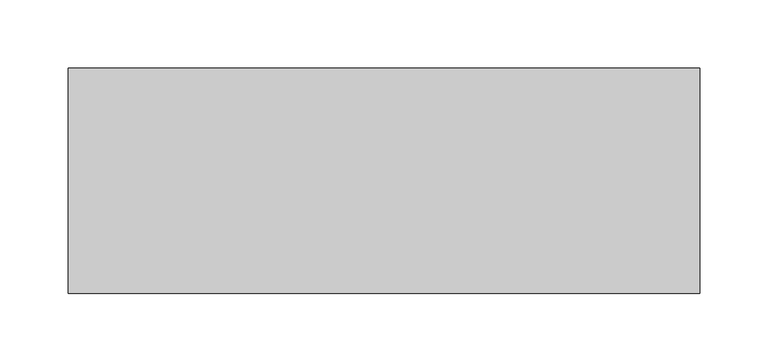
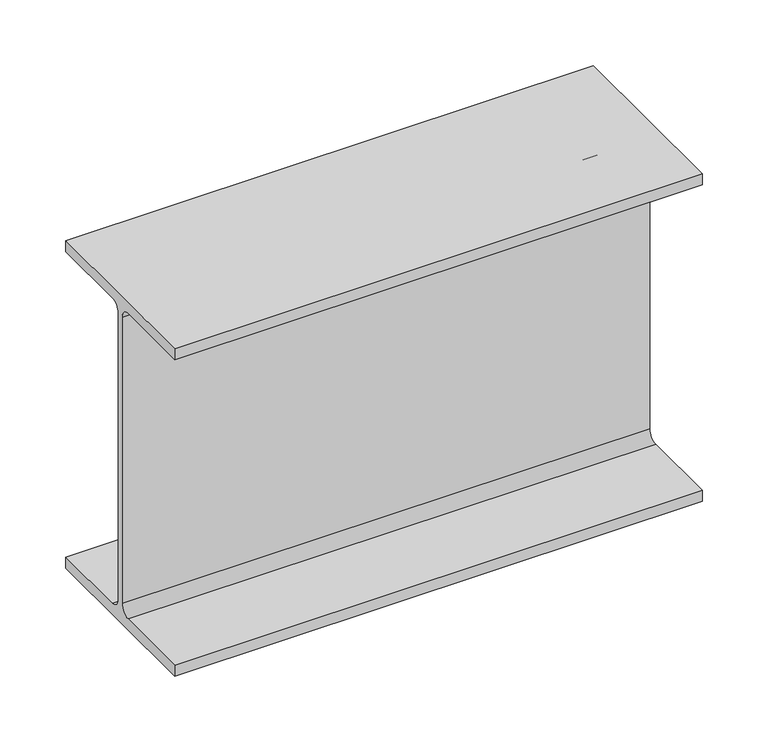
"""IFC4 building model written with IfcOpenShell, lengths in millimetres: beam geometry, Steel Beam_H-KSD3502 : H_SB_ASB_H-300x150x6.5x9."""

from ifc_helpers import new_model, si_unit, point, frame, frame_2d, origin, place, context, project, spatial, polyline, circle_curve, trimmed, segment, composite_curve, outline, extrude, source, transform, mapped, element, save


def beam_c8f6394c(model_context):
    return source(origin(), model_context, "Body", "SweptSolid", [
        extrude(outline(composite_curve([segment(polyline([(82.5, -141.5), (82.5, -151.7), (-82.5, -151.7), (-82.5, -141.5), (-11.9, -141.5)]), True, "CONTINUOUS"), segment(trimmed(circle_curve(frame_2d((-11.9, -132.6)), 8.9), [point((-11.9, -141.5))], [point((-3.0, -132.6))], True, "CARTESIAN"), True, "CONTINUOUS"), segment(polyline([(-3.0, -132.6), (-3.0, 132.6)]), True, "CONTINUOUS"), segment(trimmed(circle_curve(frame_2d((-11.9, 132.6)), 8.9), [point((-3.0, 132.6))], [point((-11.9, 141.5))], True, "CARTESIAN"), True, "CONTINUOUS"), segment(polyline([(-11.9, 141.5), (-82.5, 141.5), (-82.5, 151.7), (82.5, 151.7), (82.5, 141.5), (11.9, 141.5)]), True, "CONTINUOUS"), segment(trimmed(circle_curve(frame_2d((11.9, 132.6)), 8.9), [point((11.9, 141.5))], [point((3.0, 132.6))], True, "CARTESIAN"), True, "CONTINUOUS"), segment(polyline([(3.0, 132.6), (3.0, -132.6)]), True, "CONTINUOUS"), segment(trimmed(circle_curve(frame_2d((11.9, -132.6)), 8.9), [point((3.0, -132.6))], [point((11.9, -141.5))], True, "CARTESIAN"), True, "CONTINUOUS"), segment(polyline([(11.9, -141.5), (82.5, -141.5)]), True, "CONTINUOUS")], self_intersect=False)), frame((-300.0, 0.0, 0.0), z_axis=(1.0, 0.0, 0.0), x_axis=(0.0, 1.0, 0.0)), (0.0, 0.0, 1.0), 462.3),
    ])


if __name__ == "__main__":
    model = new_model("IFC4")
    model_context = context("Model", 3, world=origin())
    ifc_project = project(units=[si_unit("LENGTHUNIT", "METRE", prefix="MILLI")], contexts=[model_context])
    site = spatial("IfcSite", under=ifc_project)
    building = spatial("IfcBuilding", under=site)
    placement = place(None, origin())
    beam_shape = beam_c8f6394c(model_context)
    element("IfcBeam", 1, ObjectType="Steel Beam_H-KSD3502 : H_SB_ASB_H-300x150x6.5x9", at=placement, inside=building, context=model_context, shape_type="MappedRepresentation", body=[
        mapped(beam_shape, transform((0.0, 0.0, 0.0), x_axis=(1.0, 0.0, 0.0), y_axis=(0.0, 1.0, 0.0), z_axis=(0.0, 0.0, 1.0))),
    ])
    save(model, "model.ifc")

# Revit data of these elements
# Type "Steel Beam_H-KSD3502 : H_SB_ASB_H-300x150x6.5x9"
#   Width = 15.0 cm
#   Web Thickness = 0.65 cm
#   Web Fillet = 1.3 cm
#   Warping Constant = 107174.0 cm⁶
#   Torsional Moment of Inertia = 9.9539 cm⁴
#   Torsional Modulus = 1.0 cm³
#   Section Area = 46.78 cm²
#   Plastic Modulus weak axis = 105.0 cm³
#   Plastic Modulus strong axis = 542.0 cm³
#   Perimeter = 1.17 m²/m
#   Nominal Weight = 36.70 kgf/m
#   Moment of Inertia weak axis = 508.00 cm⁴
#   Moment of Inertia strong axis = 7210.00 cm⁴
#   Height = 30.0 cm
#   Flange Thickness = 0.9 cm
#   Elastic Modulus weak axis = 67.7 cm³
#   Elastic Modulus strong axis = 481.0 cm³
#   Centroid Vertical = 15.0 cm
#   Centroid Horizontal = 7.5 cm
#   Length [instance default] = 1.5240 m
#   Structural Material [instance default] = Steel, 45-345
#   Assembly Code = ""
# Element 1 (IfcBeam, "Steel Beam_H-KSD3502 : H_SB_ASB_H-300x150x6.5x9")
#   Structural Material = none
# Materials
#   "Steel, 45-345": class "Metal", colour RGB 189 187 185, transparency 0, Description = "Steel 345 MPa", Cost = 0
